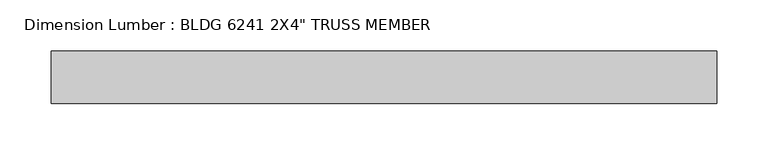
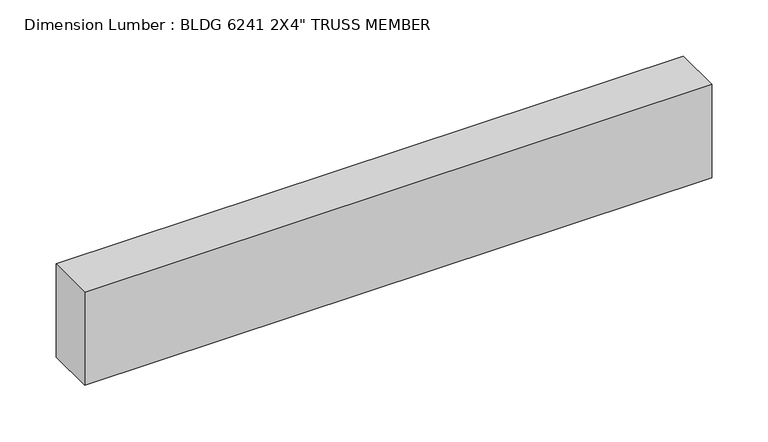
"""IFC4 building model written with IfcOpenShell, lengths in millimetres: beam geometry."""

from ifc_helpers import new_model, si_unit, frame, origin, place, context, project, spatial, polyline, outline, extrude, source, transform, mapped, element, save


def beam_29c6d41d(model_context):
    return source(origin(), model_context, "Body", "SweptSolid", [
        extrude(outline(polyline([(350.5042173, 25.4), (350.5042173, -25.4), (-295.4519367, -25.4), (-295.4519367, 25.4), (350.5042173, 25.4)])), frame((0.0, 0.0, -50.8), z_axis=(0.0, 0.0, 1.0), x_axis=(1.0, 0.0, 0.0)), (0.0, 0.0, 1.0), 101.6),
    ])


if __name__ == "__main__":
    model = new_model("IFC4")
    model_context = context("Model", 3, world=origin())
    ifc_project = project(units=[si_unit("LENGTHUNIT", "METRE", prefix="MILLI")], contexts=[model_context])
    site = spatial("IfcSite", under=ifc_project)
    building = spatial("IfcBuilding", under=site)
    placement = place(None, origin())
    beam_shape = beam_29c6d41d(model_context)
    element("IfcBeam", 1, ObjectType="Dimension Lumber : BLDG 6241 2X4\" TRUSS MEMBER", at=placement, inside=building, context=model_context, shape_type="MappedRepresentation", body=[
        mapped(beam_shape, transform((0.0, 0.0, 0.0), x_axis=(1.0, 0.0, 0.0), y_axis=(0.0, 1.0, 0.0), z_axis=(0.0, 0.0, 1.0))),
    ])
    save(model, "model.ifc")

# Revit data of these elements
# Type "Dimension Lumber : BLDG 6241 2X4\" TRUSS MEMBER"
#   Assembly Code = "B10"
#   A = 0.273472 SF
#   Length [instance default] = 5' - 0"
#   b = 0' - 2"
#   d = 0' - 4"
#   Structural Material [instance default] = Softwood, Lumber
# Element 1 (IfcBeam, "Dimension Lumber : BLDG 6241 2X4\" TRUSS MEMBER")
#   Materials on its faces: "Softwood, Lumber"
# Materials
#   "Softwood, Lumber": class "Wood", colour RGB 223 192 134, transparency 0, Description = "Pinus Echinata", Cost = 0
